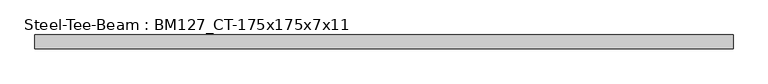
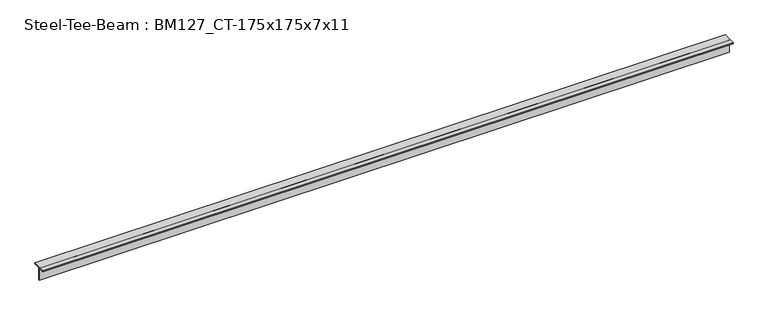
"""IFC4 building model written with IfcOpenShell, lengths in millimetres: beam geometry, Steel-Tee-Beam : BM127_CT-175x175x7x11."""

from ifc_helpers import new_model, si_unit, point, frame, frame_2d, origin, place, context, project, spatial, polyline, circle_curve, trimmed, segment, composite_curve, outline, extrude, source, transform, mapped, element, save


def steel_tee_beam_bm127_ct_175x175x7x11_fc6d57d6(model_context):
    return source(origin(), model_context, "Body", "SweptSolid", [
        extrude(outline(composite_curve([segment(polyline([(-87.5, 87.5), (87.5, 87.5), (87.5, 76.5), (17.5, 76.5)]), True, "CONTINUOUS"), segment(trimmed(circle_curve(frame_2d((17.5, 62.5)), 14.0), [point((17.5, 76.5))], [point((3.5, 62.5))], True, "CARTESIAN"), True, "CONTINUOUS"), segment(polyline([(3.5, 62.5), (3.5, -87.5), (-3.5, -87.5), (-3.5, 62.5)]), True, "CONTINUOUS"), segment(trimmed(circle_curve(frame_2d((-17.5, 62.5)), 14.0), [point((-3.5, 62.5))], [point((-17.5, 76.5))], True, "CARTESIAN"), True, "CONTINUOUS"), segment(polyline([(-17.5, 76.5), (-87.5, 76.5), (-87.5, 87.5)]), True, "CONTINUOUS")], self_intersect=False)), frame((-4298.1792655, 0.0, 0.0), z_axis=(1.0, 0.0, 0.0), x_axis=(0.0, 1.0, 0.0)), (0.0, 0.0, 1.0), 8725.555017),
    ])


if __name__ == "__main__":
    model = new_model("IFC4")
    model_context = context("Model", 3, world=origin())
    ifc_project = project(units=[si_unit("LENGTHUNIT", "METRE", prefix="MILLI")], contexts=[model_context])
    site = spatial("IfcSite", under=ifc_project)
    building = spatial("IfcBuilding", under=site)
    placement = place(None, origin())
    steel_tee_beam_bm127_ct_175x175x7x11_shape = steel_tee_beam_bm127_ct_175x175x7x11_fc6d57d6(model_context)
    element("IfcBeam", 1, ObjectType="Steel-Tee-Beam : BM127_CT-175x175x7x11", at=placement, inside=building, context=model_context, shape_type="MappedRepresentation", body=[
        mapped(steel_tee_beam_bm127_ct_175x175x7x11_shape, transform((0.0, 0.0, 0.0), x_axis=(1.0, 0.0, 0.0), y_axis=(0.0, 1.0, 0.0), z_axis=(0.0, 0.0, 1.0))),
    ])
    save(model, "model.ifc")

# Revit data of these elements
# Type "Steel-Tee-Beam : BM127_CT-175x175x7x11"
#   Section Area = 31.57 cm²
#   Mass per Unit Length = 24.80 kg/m
#   Length [instance default] = 1524 mm
#   bf = 175 mm
#   d = 175 mm
#   k = 25 mm
#   kr = 14 mm
#   tf = 11 mm
#   tw = 7 mm
#   hec_material4 [instance default] = none
#   hec_material3 [instance default] = none
#   hec_material2 [instance default] = none
#   hec_material1 [instance default] = none
#   Structural Material [instance default] = Steel, 45-345
#   Assembly Code = ""
# Element 1 (IfcBeam, "Steel-Tee-Beam : BM127_CT-175x175x7x11")
#   hec_material3 = F01AC000-00002_Building/Shelter Fire Proofing Work_Intumescent Coating Type_1 hr. rating (UL 1709))
#   hec_material1 = S03AA029-00001_Main Steel Structure Erection Work_Shelter/Building_Light Steel
#   Structural Material = S01AA003-00001_Main Steel Structure Fabrication Work_Shelter/Building_Light Steel - Standard
#   Materials on its faces: "S01AA003-00001_Main Steel Structure Fabrication Work_Shelter/Building_Light Steel - Standard"
# Materials
#   "Steel, 45-345": class "Metal", colour RGB 189 187 185, transparency 0, Description = "Steel 345 MPa", Cost = 0
#   "S01AA003-00001_Main Steel Structure Fabrication Work_Shelter/Building_Light Steel - Standard": class "Metal", colour RGB 120 120 120, transparency 0, Comments = "(30KG/M>Weight)", Description = "Structural steel 50ksi", W00) Work Master Code = "S01AA003-00001", W01) Work Master_Lv1 = "Main Steel Structure Fabrication Work", W02) Work Master_Lv2 = "Shelter/Building", W03) Work Master_Spec.1 = "Light Steel - Standard (30KG/M>Weight)", Cost = 0
#   "F01AC000-00002_Building/Shelter Fire Proofing Work_Intumescent Coating Type_1 hr. rating (UL 1709))": class "Metal", colour RGB 255 128 128, transparency 0, Description = "Paint finished steel", W00) Work Master Code = "F01AC000-00002", W01) Work Master_Lv1 = "Building/Shelter Fire Proofing Work", W02) Work Master_Lv2 = "Intumescent Coating Type", W03) Work Master_Spec.1 = "1 hr. rating (UL 1709)", Cost = 0
#   "S03AA029-00001_Main Steel Structure Erection Work_Shelter/Building_Light Steel": class "Metal", colour RGB 120 120 120, transparency 0, Comments = "(30KG/M>Weight)", Description = "Structural steel 50ksi", W00) Work Master Code = "S03AA029-00001", W01) Work Master_Lv1 = "Main Steel Structure Erection Work", W02) Work Master_Lv2 = "Shelter/Building", W03) Work Master_Spec.1 = "Light Steel (30KG/M>Weight)", Cost = 0
